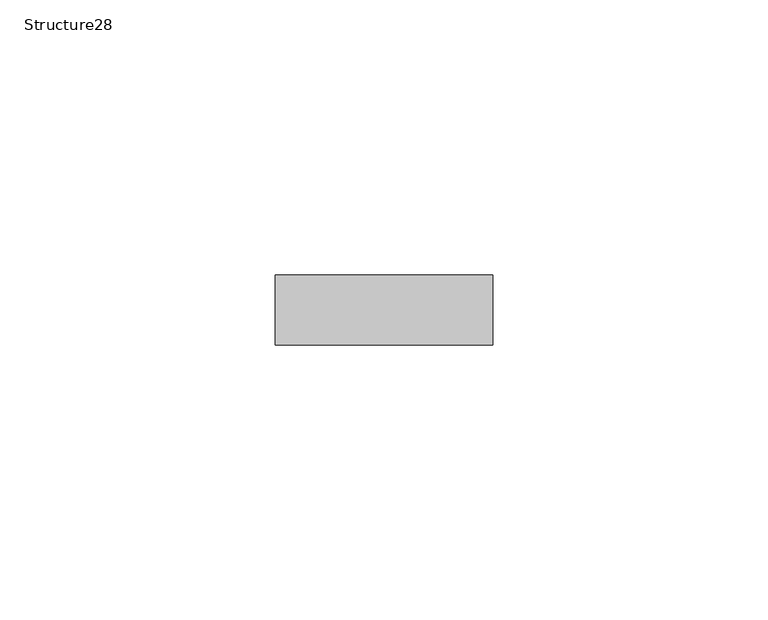
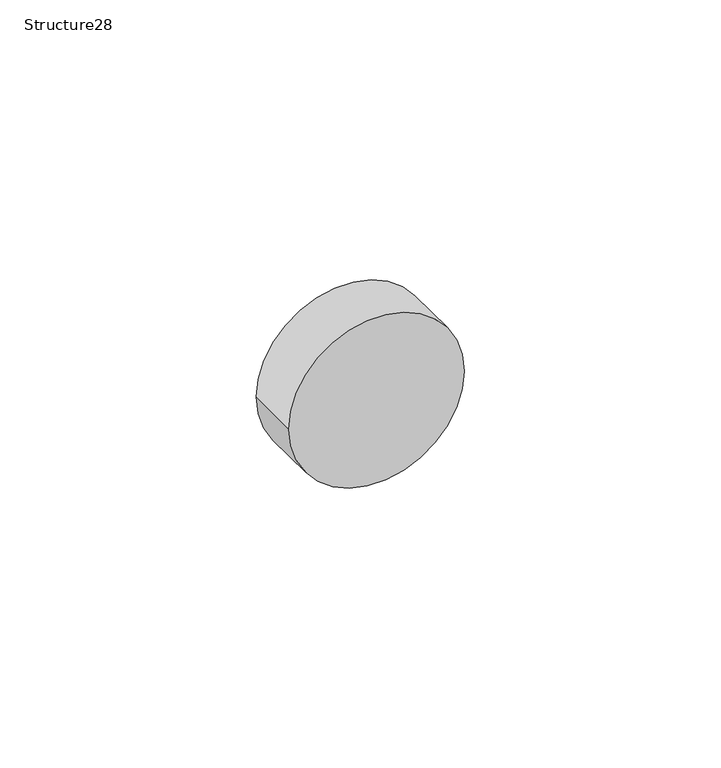
"""IFC4 building model written with IfcOpenShell, lengths in millimetres: proxy geometry, Structure28 : Structure668217126."""

from ifc_helpers import new_model, si_unit, point, frame, frame_2d, origin, place, context, project, spatial, circle_curve, trimmed, segment, composite_curve, outline, extrude, source, transform, mapped, element, save


def structure28_e75c90f0(model_context):
    return source(origin(), model_context, "Body", "SweptSolid", [
        extrude(outline(composite_curve([segment(trimmed(circle_curve(frame_2d((39371.6422813, 7343.0332877)), 19.7708678), [point((39371.6422813, 7323.2624199))], [point((39371.6422813, 7362.8041555))], False, "CARTESIAN"), True, "CONTINUOUS"), segment(trimmed(circle_curve(frame_2d((39371.6422813, 7343.0332877)), 19.7708678), [point((39371.6422813, 7362.8041555))], [point((39371.6422813, 7323.2624199))], False, "CARTESIAN"), True, "CONTINUOUS")], self_intersect=False)), frame((0.0, 870.0121669, 0.0), z_axis=(0.0, 1.0, 0.0), x_axis=(0.0, 0.0, 1.0)), (0.0, 0.0, 1.0), 12.7),
    ])


if __name__ == "__main__":
    model = new_model("IFC4")
    model_context = context("Model", 3, world=origin())
    ifc_project = project(units=[si_unit("LENGTHUNIT", "METRE", prefix="MILLI")], contexts=[model_context])
    site = spatial("IfcSite", under=ifc_project)
    building = spatial("IfcBuilding", under=site)
    placement = place(None, origin())
    structure28_shape = structure28_e75c90f0(model_context)
    element("IfcBuildingElementProxy", 1, Name="Structure28 : Structure668217126", ObjectType="Structure28 : Structure668217126", at=placement, inside=building, context=model_context, shape_type="MappedRepresentation", body=[
        mapped(structure28_shape, transform((0.0, 0.0, 0.0), x_axis=(1.0, 0.0, 0.0), y_axis=(0.0, 1.0, 0.0), z_axis=(0.0, 0.0, 1.0))),
    ])
    save(model, "model.ifc")

# Revit data of these elements
# Type "Structure28 : Structure668217126"
#   NameOverride = "Structure668217126"
# Element 1 (IfcBuildingElementProxy, "Structure28 : Structure668217126")
#   Materials on its faces: "1.5\" DIA. STAINLESS STEEL RAILING"
# Materials
#   "1.5\" DIA. STAINLESS STEEL RAILING": class "Unassigned", colour RGB 128 128 128, transparency 0, Cost = 0
